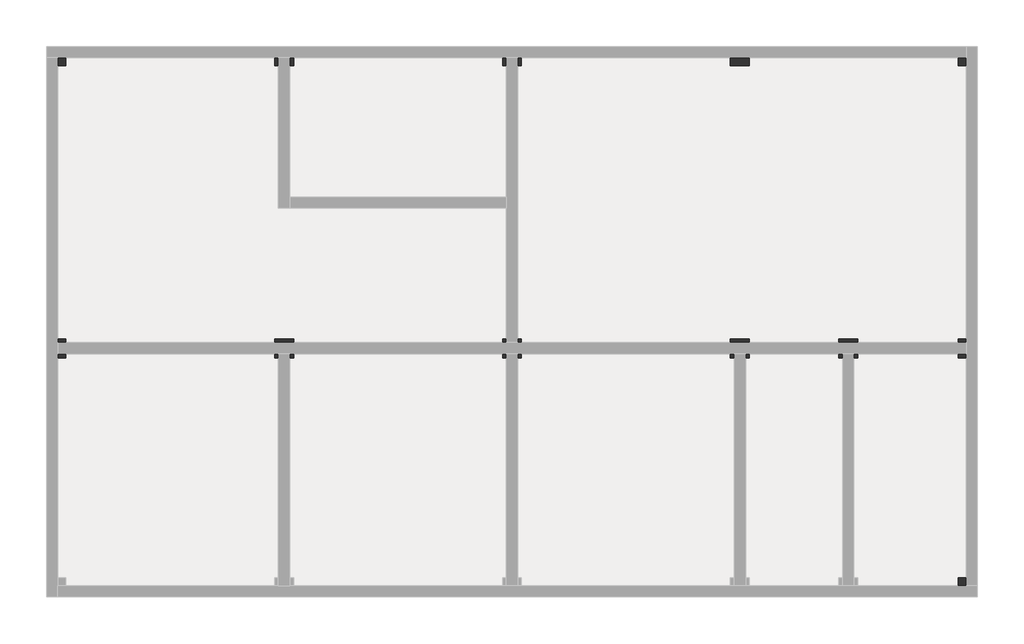
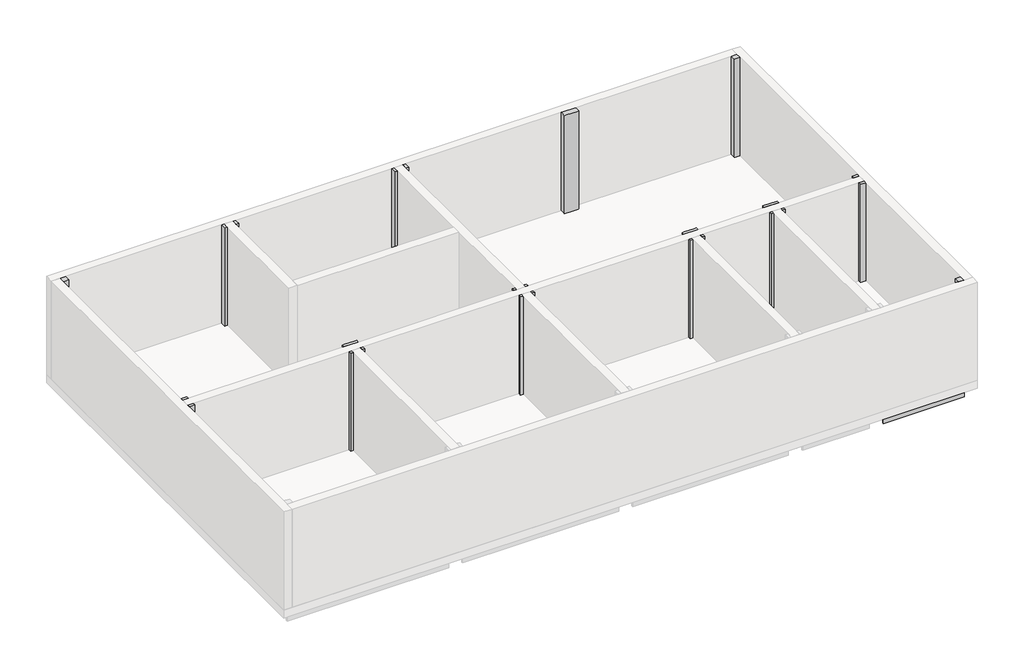
# One storey, part 2 of 2: 17 beams, 12 columns.
"""IFC4 building model written with IfcOpenShell, lengths in millimetres."""

from ifc_helpers import new_model, si_unit, frame, origin, place, context, project, spatial, polyline, outline, extrude, faceted_brep, element, save

model = new_model("IFC4")

# Units and contexts
model_context = context("Model", 3, world=origin())
ifc_project = project(units=[si_unit("LENGTHUNIT", "METRE", prefix="MILLI")], contexts=[model_context])

# Site, building, storey
site = spatial("IfcSite", under=ifc_project)
building = spatial("IfcBuilding", under=site)
storey = spatial("IfcBuildingStorey", under=building, Name="2nd FL GL+6,200", Elevation=6000.0)

# Beams
placement = place(None, origin())
element("IfcBeam", 1, ObjectType="RC Beam_Rectangular : 350 x 700mm", at=placement, inside=storey, context=model_context, shape_type="SweptSolid", body=[
    extrude(outline(polyline([(-18645.7273237, 9185.9763125), (-18595.7273237, 9185.9763125), (-18595.7273237, 1985.9763125), (-18645.7273237, 1985.9763125), (-18645.7273237, 9185.9763125)])), frame((0.0, 0.0, 5300.0), z_axis=(0.0, 0.0, 1.0), x_axis=(1.0, 0.0, 0.0)), (0.0, 0.0, 1.0), 400.0),
])
element("IfcBeam", 2, ObjectType="RC Beam_Rectangular : 350 x 700mm", at=placement, inside=storey, context=model_context, shape_type="SweptSolid", body=[
    extrude(outline(polyline([(-12870.7273237, 9185.9763125), (-12520.7273237, 9185.9763125), (-12520.7273237, 1985.9763125), (-12870.7273237, 1985.9763125), (-12870.7273237, 9185.9763125)])), frame((0.0, 0.0, 5300.0), z_axis=(0.0, 0.0, 1.0), x_axis=(1.0, 0.0, 0.0)), (0.0, 0.0, 1.0), 400.0),
])
element("IfcBeam", 3, ObjectType="RC Beam_Rectangular : 350 x 700mm", at=placement, inside=storey, context=model_context, shape_type="SweptSolid", body=[
    extrude(outline(polyline([(-6870.7273237, 9185.9763125), (-6520.7273237, 9185.9763125), (-6520.7273237, 1985.9763125), (-6870.7273237, 1985.9763125), (-6870.7273237, 9185.9763125)])), frame((0.0, 0.0, 5300.0), z_axis=(0.0, 0.0, 1.0), x_axis=(1.0, 0.0, 0.0)), (0.0, 0.0, 1.0), 400.0),
])
element("IfcBeam", 4, ObjectType="RC Beam_Rectangular : 350 x 700mm", at=placement, inside=storey, context=model_context, shape_type="SweptSolid", body=[
    extrude(outline(polyline([(-870.7273237, 9185.9763125), (-520.7273237, 9185.9763125), (-520.7273237, 1985.9763125), (-870.7273237, 1985.9763125), (-870.7273237, 9185.9763125)])), frame((0.0, 0.0, 5300.0), z_axis=(0.0, 0.0, 1.0), x_axis=(1.0, 0.0, 0.0)), (0.0, 0.0, 1.0), 400.0),
])
element("IfcBeam", 5, ObjectType="RC Beam_Rectangular : 350 x 700mm", at=placement, inside=storey, context=model_context, shape_type="SweptSolid", body=[
    extrude(outline(polyline([(5204.2726763, 1485.9763125), (5254.2726763, 1485.9763125), (5254.2726763, -4314.0236875), (5204.2726763, -4314.0236875), (5204.2726763, 1485.9763125)])), frame((0.0, 0.0, 5300.0), z_axis=(0.0, 0.0, 1.0), x_axis=(1.0, 0.0, 0.0)), (0.0, 0.0, 1.0), 400.0),
])
element("IfcBeam", 6, ObjectType="RC Beam_Rectangular : 350 x 700mm", at=placement, inside=storey, context=model_context, shape_type="SweptSolid", body=[
    extrude(outline(polyline([(5204.2726763, 9185.9763125), (5254.2726763, 9185.9763125), (5254.2726763, 1885.9763125), (5204.2726763, 1885.9763125), (5204.2726763, 9185.9763125)])), frame((0.0, 0.0, 5300.0), z_axis=(0.0, 0.0, 1.0), x_axis=(1.0, 0.0, 0.0)), (0.0, 0.0, 1.0), 400.0),
])
element("IfcBeam", 7, ObjectType="RC Beam_Rectangular : 350 x 700mm", at=placement, inside=storey, context=model_context, shape_type="SweptSolid", body=[
    extrude(outline(polyline([(-12945.7273237, 9385.9763125), (-12945.7273237, 9335.9763125), (-18645.7273237, 9335.9763125), (-18645.7273237, 9385.9763125), (-12945.7273237, 9385.9763125)])), frame((0.0, 0.0, 5300.0), z_axis=(0.0, 0.0, 1.0), x_axis=(1.0, 0.0, 0.0)), (0.0, 0.0, 1.0), 400.0),
])
element("IfcBeam", 8, ObjectType="RC Beam_Rectangular : 350 x 700mm", at=placement, inside=storey, context=model_context, shape_type="SweptSolid", body=[
    extrude(outline(polyline([(-12445.7273237, 9335.9763125), (-12445.7273237, 9385.9763125), (-6945.7273237, 9385.9763125), (-6945.7273237, 9335.9763125), (-12445.7273237, 9335.9763125)])), frame((0.0, 0.0, 5300.0), z_axis=(0.0, 0.0, 1.0), x_axis=(1.0, 0.0, 0.0)), (0.0, 0.0, 1.0), 400.0),
])
element("IfcBeam", 9, ObjectType="RC Beam_Rectangular : 350 x 700mm", at=placement, inside=storey, context=model_context, shape_type="SweptSolid", body=[
    extrude(outline(polyline([(-6445.7273237, 9335.9763125), (-6445.7273237, 9385.9763125), (-945.7273237, 9385.9763125), (-945.7273237, 9335.9763125), (-6445.7273237, 9335.9763125)])), frame((0.0, 0.0, 5300.0), z_axis=(0.0, 0.0, 1.0), x_axis=(1.0, 0.0, 0.0)), (0.0, 0.0, 1.0), 400.0),
])
element("IfcBeam", 10, ObjectType="RC Beam_Rectangular : 350 x 700mm", at=placement, inside=storey, context=model_context, shape_type="SweptSolid", body=[
    extrude(outline(polyline([(-433.0273237, 9385.9763125), (5254.2726763, 9385.9763125), (5254.2726763, 9335.9763125), (-433.0273237, 9335.9763125), (-433.0273237, 9385.9763125)])), frame((0.0, 0.0, 5300.0), z_axis=(0.0, 0.0, 1.0), x_axis=(1.0, 0.0, 0.0)), (0.0, 0.0, 1.0), 400.0),
])
element("IfcBeam", 11, ObjectType="RC Beam_Rectangular : 350 x 700mm", at=placement, inside=storey, context=model_context, shape_type="SweptSolid", body=[
    extrude(outline(polyline([(-18445.7273237, 1560.9763125), (-18445.7273237, 1585.9763125), (-12945.7273237, 1585.9763125), (-12945.7273237, 1560.9763125), (-18445.7273237, 1560.9763125)])), frame((0.0, 0.0, 5300.0), z_axis=(0.0, 0.0, 1.0), x_axis=(1.0, 0.0, 0.0)), (0.0, 0.0, 1.0), 400.0),
    extrude(outline(polyline([(-18445.7273237, 1885.9763125), (-18445.7273237, 1910.9763125), (-12945.7273237, 1910.9763125), (-12945.7273237, 1885.9763125), (-18445.7273237, 1885.9763125)])), frame((0.0, 0.0, 5300.0), z_axis=(0.0, 0.0, 1.0), x_axis=(1.0, 0.0, 0.0)), (0.0, 0.0, 1.0), 400.0),
])
element("IfcBeam", 12, ObjectType="RC Beam_Rectangular : 350 x 700mm", at=placement, inside=storey, context=model_context, shape_type="SweptSolid", body=[
    extrude(outline(polyline([(-12445.7273237, 1560.9763125), (-12445.7273237, 1585.9763125), (-6945.7273237, 1585.9763125), (-6945.7273237, 1560.9763125), (-12445.7273237, 1560.9763125)])), frame((0.0, 0.0, 5300.0), z_axis=(0.0, 0.0, 1.0), x_axis=(1.0, 0.0, 0.0)), (0.0, 0.0, 1.0), 400.0),
    extrude(outline(polyline([(-12445.7273237, 1885.9763125), (-12445.7273237, 1910.9763125), (-6945.7273237, 1910.9763125), (-6945.7273237, 1885.9763125), (-12445.7273237, 1885.9763125)])), frame((0.0, 0.0, 5300.0), z_axis=(0.0, 0.0, 1.0), x_axis=(1.0, 0.0, 0.0)), (0.0, 0.0, 1.0), 400.0),
])
element("IfcBeam", 13, ObjectType="RC Beam_Rectangular : 350 x 700mm", at=placement, inside=storey, context=model_context, shape_type="SweptSolid", body=[
    extrude(outline(polyline([(-6445.7273237, 1560.9763125), (-6445.7273237, 1585.9763125), (-945.7273237, 1585.9763125), (-945.7273237, 1560.9763125), (-6445.7273237, 1560.9763125)])), frame((0.0, 0.0, 5300.0), z_axis=(0.0, 0.0, 1.0), x_axis=(1.0, 0.0, 0.0)), (0.0, 0.0, 1.0), 400.0),
    extrude(outline(polyline([(-6445.7273237, 1885.9763125), (-6445.7273237, 1910.9763125), (-945.7273237, 1910.9763125), (-945.7273237, 1885.9763125), (-6445.7273237, 1885.9763125)])), frame((0.0, 0.0, 5300.0), z_axis=(0.0, 0.0, 1.0), x_axis=(1.0, 0.0, 0.0)), (0.0, 0.0, 1.0), 400.0),
])
element("IfcBeam", 14, ObjectType="RC Beam_Rectangular : 350 x 700mm", at=placement, inside=storey, context=model_context, shape_type="SweptSolid", body=[
    extrude(outline(polyline([(-445.7273237, 1560.9763125), (-445.7273237, 1585.9763125), (1904.2726763, 1585.9763125), (1904.2726763, 1560.9763125), (-445.7273237, 1560.9763125)])), frame((0.0, 0.0, 5300.0), z_axis=(0.0, 0.0, 1.0), x_axis=(1.0, 0.0, 0.0)), (0.0, 0.0, 1.0), 400.0),
    extrude(outline(polyline([(-445.7273237, 1885.9763125), (-445.7273237, 1910.9763125), (1904.2726763, 1910.9763125), (1904.2726763, 1885.9763125), (-445.7273237, 1885.9763125)])), frame((0.0, 0.0, 5300.0), z_axis=(0.0, 0.0, 1.0), x_axis=(1.0, 0.0, 0.0)), (0.0, 0.0, 1.0), 400.0),
])
element("IfcBeam", 15, ObjectType="RC Beam_Rectangular : 350 x 700mm", at=placement, inside=storey, context=model_context, shape_type="SweptSolid", body=[
    extrude(outline(polyline([(5054.2726763, 1585.9763125), (5054.2726763, 1560.9763125), (2404.2726763, 1560.9763125), (2404.2726763, 1585.9763125), (5054.2726763, 1585.9763125)])), frame((0.0, 0.0, 5300.0), z_axis=(0.0, 0.0, 1.0), x_axis=(1.0, 0.0, 0.0)), (0.0, 0.0, 1.0), 400.0),
    extrude(outline(polyline([(5054.2726763, 1910.9763125), (5054.2726763, 1885.9763125), (2404.2726763, 1885.9763125), (2404.2726763, 1910.9763125), (5054.2726763, 1910.9763125)])), frame((0.0, 0.0, 5300.0), z_axis=(0.0, 0.0, 1.0), x_axis=(1.0, 0.0, 0.0)), (0.0, 0.0, 1.0), 400.0),
])
element("IfcBeam", 16, ObjectType="RC Beam_Rectangular : 350 x 700mm", at=placement, inside=storey, context=model_context, shape_type="SweptSolid", body=[
    extrude(outline(polyline([(2404.2726763, -4514.0236875), (2404.2726763, -4464.0236875), (5254.2726763, -4464.0236875), (5254.2726763, -4514.0236875), (2404.2726763, -4514.0236875)])), frame((0.0, 0.0, 5300.0), z_axis=(0.0, 0.0, 1.0), x_axis=(1.0, 0.0, 0.0)), (0.0, 0.0, 1.0), 400.0),
])
element("IfcBeam", 17, ObjectType="RC Beam_Rectangular : 350 x 700mm", at=placement, inside=storey, context=model_context, shape_type="SweptSolid", body=[
    extrude(outline(polyline([(2304.2726763, 1485.9763125), (2329.2726763, 1485.9763125), (2329.2726763, -4314.0236875), (2304.2726763, -4314.0236875), (2304.2726763, 1485.9763125)])), frame((0.0, 0.0, 5300.0), z_axis=(0.0, 0.0, 1.0), x_axis=(1.0, 0.0, 0.0)), (0.0, 0.0, 1.0), 400.0),
    extrude(outline(polyline([(1979.2726763, 1485.9763125), (2004.2726763, 1485.9763125), (2004.2726763, -4314.0236875), (1979.2726763, -4314.0236875), (1979.2726763, 1485.9763125)])), frame((0.0, 0.0, 5300.0), z_axis=(0.0, 0.0, 1.0), x_axis=(1.0, 0.0, 0.0)), (0.0, 0.0, 1.0), 400.0),
])

# Columns
element("IfcColumn", 18, ObjectType="RC_Column_Rectangular : 500 x 500mm", at=placement, inside=storey, context=model_context, shape_type="Brep", body=[
    faceted_brep([(-18445.7273237, 9385.9763125, 6000.0), (-18445.7273237, 9185.9763125, 6000.0), (-18645.7273237, 9185.9763125, 6000.0), (-18645.7273237, 9385.9763125, 6000.0), (-18445.7273237, 9185.9763125, 9667.0), (-18595.7273237, 9185.9763125, 9667.0), (-18645.7273237, 9185.9763125, 9667.0), (-18645.7273237, 9185.9763125, 9300.0), (-18445.7273237, 9385.9763125, 9300.0), (-18445.7273237, 9385.9763125, 9667.0), (-18445.7273237, 9335.9763125, 9667.0), (-18645.7273237, 9385.9763125, 9667.0)], [[[0, 1, 2, 3]], [[1, 4, 5, 6, 7, 2]], [[4, 1, 0, 8, 9, 10]], [[4, 10, 9, 11, 6, 5]], [[9, 8, 0, 3, 11]], [[3, 2, 7, 6, 11]]]),
])
element("IfcColumn", 19, ObjectType="RC_Column_Rectangular : 500 x 500mm", at=placement, inside=storey, context=model_context, shape_type="Brep", body=[
    faceted_brep([(-18645.7273237, 1985.9763125, 6000.0), (-18445.7273237, 1985.9763125, 6000.0), (-18445.7273237, 1885.9763125, 6000.0), (-18645.7273237, 1885.9763125, 6000.0), (-18445.7273237, 1985.9763125, 9667.0), (-18645.7273237, 1985.9763125, 9300.0), (-18645.7273237, 1985.9763125, 9667.0), (-18595.7273237, 1985.9763125, 9667.0), (-18445.7273237, 1910.9763125, 9667.0), (-18445.7273237, 1885.9763125, 9667.0), (-18445.7273237, 1885.9763125, 9300.0), (-18645.7273237, 1885.9763125, 9667.0)], [[[0, 1, 2, 3]], [[4, 1, 0, 5, 6, 7]], [[1, 4, 8, 9, 10, 2]], [[4, 7, 6, 11, 9, 8]], [[3, 2, 10, 9, 11]], [[6, 5, 0, 3, 11]]]),
    faceted_brep([(-18445.7273237, 1485.9763125, 6000.0), (-18445.7273237, 1485.9763125, 9667.0), (-18595.7273237, 1485.9763125, 9667.0), (-18645.7273237, 1485.9763125, 9667.0), (-18645.7273237, 1485.9763125, 9300.0), (-18645.7273237, 1485.9763125, 6000.0), (-18645.7273237, 1585.9763125, 9667.0), (-18645.7273237, 1585.9763125, 6000.0), (-18445.7273237, 1585.9763125, 6000.0), (-18445.7273237, 1585.9763125, 9667.0), (-18445.7273237, 1585.9763125, 9300.0), (-18445.7273237, 1560.9763125, 9667.0)], [[[0, 1, 2, 3, 4, 5]], [[5, 4, 3, 6, 7]], [[8, 7, 6, 9, 10]], [[0, 5, 7, 8]], [[1, 0, 8, 10, 9, 11]], [[3, 2, 1, 11, 9, 6]]]),
])
element("IfcColumn", 20, ObjectType="RC_Column_Rectangular : 500 x 500mm", at=placement, inside=storey, context=model_context, shape_type="Brep", body=[
    faceted_brep([(-12945.7273237, 9185.9763125, 6000.0), (-12945.7273237, 9385.9763125, 6000.0), (-12845.7273237, 9385.9763125, 6000.0), (-12845.7273237, 9185.9763125, 6000.0), (-12945.7273237, 9185.9763125, 9667.0), (-12945.7273237, 9335.9763125, 9667.0), (-12945.7273237, 9385.9763125, 9667.0), (-12945.7273237, 9385.9763125, 9300.0), (-12845.7273237, 9185.9763125, 9300.0), (-12845.7273237, 9185.9763125, 9667.0), (-12870.7273237, 9185.9763125, 9667.0), (-12845.7273237, 9385.9763125, 9667.0)], [[[0, 1, 2, 3]], [[0, 4, 5, 6, 7, 1]], [[4, 0, 3, 8, 9, 10]], [[6, 5, 4, 10, 9, 11]], [[1, 7, 6, 11, 2]], [[3, 2, 11, 9, 8]]]),
    faceted_brep([(-12445.7273237, 9185.9763125, 9667.0), (-12445.7273237, 9185.9763125, 6000.0), (-12445.7273237, 9385.9763125, 6000.0), (-12445.7273237, 9385.9763125, 9300.0), (-12445.7273237, 9385.9763125, 9667.0), (-12445.7273237, 9335.9763125, 9667.0), (-12545.7273237, 9385.9763125, 6000.0), (-12545.7273237, 9185.9763125, 6000.0), (-12545.7273237, 9185.9763125, 9300.0), (-12545.7273237, 9185.9763125, 9667.0), (-12545.7273237, 9385.9763125, 9667.0), (-12520.7273237, 9185.9763125, 9667.0)], [[[0, 1, 2, 3, 4, 5]], [[6, 7, 8, 9, 10]], [[2, 1, 7, 6]], [[1, 0, 11, 9, 8, 7]], [[0, 5, 4, 10, 9, 11]], [[4, 3, 2, 6, 10]]]),
])
element("IfcColumn", 21, ObjectType="RC_Column_Rectangular : 500 x 500mm", at=placement, inside=storey, context=model_context, shape_type="Brep", body=[
    faceted_brep([(-12945.7273237, 1985.9763125, 6000.0), (-12445.7273237, 1985.9763125, 6000.0), (-12445.7273237, 1885.9763125, 6000.0), (-12945.7273237, 1885.9763125, 6000.0), (-12945.7273237, 1985.9763125, 9667.0), (-12870.7273237, 1985.9763125, 9667.0), (-12520.7273237, 1985.9763125, 9667.0), (-12445.7273237, 1985.9763125, 9667.0), (-12945.7273237, 1885.9763125, 9300.0), (-12945.7273237, 1885.9763125, 9667.0), (-12945.7273237, 1910.9763125, 9667.0), (-12445.7273237, 1910.9763125, 9667.0), (-12445.7273237, 1885.9763125, 9667.0), (-12445.7273237, 1885.9763125, 9300.0)], [[[0, 1, 2, 3]], [[1, 0, 4, 5, 6, 7]], [[4, 0, 3, 8, 9, 10]], [[1, 7, 11, 12, 13, 2]], [[7, 6, 5, 4, 10, 9, 12, 11]], [[3, 2, 13, 12, 9, 8]]]),
    faceted_brep([(-12945.7273237, 1485.9763125, 9667.0), (-12945.7273237, 1485.9763125, 6000.0), (-12845.7273237, 1485.9763125, 6000.0), (-12845.7273237, 1485.9763125, 9300.0), (-12845.7273237, 1485.9763125, 9667.0), (-12870.7273237, 1485.9763125, 9667.0), (-12945.7273237, 1585.9763125, 6000.0), (-12945.7273237, 1585.9763125, 9300.0), (-12945.7273237, 1585.9763125, 9667.0), (-12845.7273237, 1585.9763125, 9667.0), (-12845.7273237, 1585.9763125, 6000.0), (-12945.7273237, 1560.9763125, 9667.0)], [[[0, 1, 2, 3, 4, 5]], [[6, 7, 8, 9, 10]], [[1, 6, 10, 2]], [[1, 0, 11, 8, 7, 6]], [[8, 11, 0, 5, 4, 9]], [[4, 3, 2, 10, 9]]]),
    faceted_brep([(-12445.7273237, 1485.9763125, 9667.0), (-12445.7273237, 1485.9763125, 6000.0), (-12445.7273237, 1585.9763125, 6000.0), (-12445.7273237, 1585.9763125, 9300.0), (-12445.7273237, 1585.9763125, 9667.0), (-12445.7273237, 1560.9763125, 9667.0), (-12545.7273237, 1485.9763125, 6000.0), (-12545.7273237, 1485.9763125, 9300.0), (-12545.7273237, 1485.9763125, 9667.0), (-12545.7273237, 1585.9763125, 9667.0), (-12545.7273237, 1585.9763125, 6000.0), (-12520.7273237, 1485.9763125, 9667.0)], [[[0, 1, 2, 3, 4, 5]], [[6, 7, 8, 9, 10]], [[1, 0, 11, 8, 7, 6]], [[4, 3, 2, 10, 9]], [[2, 1, 6, 10]], [[0, 5, 4, 9, 8, 11]]]),
])
element("IfcColumn", 22, ObjectType="RC_Column_Rectangular : 500 x 500mm", at=placement, inside=storey, context=model_context, shape_type="Brep", body=[
    faceted_brep([(-6945.7273237, 9185.9763125, 6000.0), (-6945.7273237, 9385.9763125, 6000.0), (-6845.7273237, 9385.9763125, 6000.0), (-6845.7273237, 9185.9763125, 6000.0), (-6945.7273237, 9185.9763125, 9667.0), (-6945.7273237, 9335.9763125, 9667.0), (-6945.7273237, 9385.9763125, 9667.0), (-6945.7273237, 9385.9763125, 9300.0), (-6845.7273237, 9185.9763125, 9300.0), (-6845.7273237, 9185.9763125, 9667.0), (-6870.7273237, 9185.9763125, 9667.0), (-6845.7273237, 9385.9763125, 9667.0)], [[[0, 1, 2, 3]], [[0, 4, 5, 6, 7, 1]], [[4, 0, 3, 8, 9, 10]], [[6, 5, 4, 10, 9, 11]], [[1, 7, 6, 11, 2]], [[3, 2, 11, 9, 8]]]),
    faceted_brep([(-6445.7273237, 9185.9763125, 9667.0), (-6445.7273237, 9185.9763125, 6000.0), (-6445.7273237, 9385.9763125, 6000.0), (-6445.7273237, 9385.9763125, 9300.0), (-6445.7273237, 9385.9763125, 9667.0), (-6445.7273237, 9335.9763125, 9667.0), (-6545.7273237, 9385.9763125, 6000.0), (-6545.7273237, 9185.9763125, 6000.0), (-6545.7273237, 9185.9763125, 9300.0), (-6545.7273237, 9185.9763125, 9667.0), (-6545.7273237, 9385.9763125, 9667.0), (-6520.7273237, 9185.9763125, 9667.0)], [[[0, 1, 2, 3, 4, 5]], [[6, 7, 8, 9, 10]], [[2, 1, 7, 6]], [[1, 0, 11, 9, 8, 7]], [[0, 5, 4, 10, 9, 11]], [[4, 3, 2, 6, 10]]]),
])
element("IfcColumn", 23, ObjectType="RC_Column_Rectangular : 500 x 500mm", at=placement, inside=storey, context=model_context, shape_type="Brep", body=[
    faceted_brep([(-6945.7273237, 1985.9763125, 6000.0), (-6845.7273237, 1985.9763125, 6000.0), (-6845.7273237, 1885.9763125, 6000.0), (-6945.7273237, 1885.9763125, 6000.0), (-6945.7273237, 1985.9763125, 9667.0), (-6945.7273237, 1885.9763125, 9300.0), (-6945.7273237, 1885.9763125, 9667.0), (-6945.7273237, 1910.9763125, 9667.0), (-6845.7273237, 1985.9763125, 9667.0), (-6870.7273237, 1985.9763125, 9667.0), (-6845.7273237, 1885.9763125, 9667.0), (-6845.7273237, 1985.9763125, 9300.0)], [[[0, 1, 2, 3]], [[4, 0, 3, 5, 6, 7]], [[8, 9, 4, 7, 6, 10]], [[2, 1, 11, 8, 10]], [[0, 4, 9, 8, 11, 1]], [[3, 2, 10, 6, 5]]]),
    faceted_brep([(-6445.7273237, 1985.9763125, 9667.0), (-6445.7273237, 1985.9763125, 6000.0), (-6545.7273237, 1985.9763125, 6000.0), (-6545.7273237, 1985.9763125, 9300.0), (-6545.7273237, 1985.9763125, 9667.0), (-6520.7273237, 1985.9763125, 9667.0), (-6445.7273237, 1910.9763125, 9667.0), (-6445.7273237, 1885.9763125, 9667.0), (-6445.7273237, 1885.9763125, 9300.0), (-6445.7273237, 1885.9763125, 6000.0), (-6545.7273237, 1885.9763125, 6000.0), (-6545.7273237, 1885.9763125, 9667.0)], [[[0, 1, 2, 3, 4, 5]], [[1, 0, 6, 7, 8, 9]], [[2, 10, 11, 4, 3]], [[10, 9, 8, 7, 11]], [[2, 1, 9, 10]], [[0, 5, 4, 11, 7, 6]]]),
    faceted_brep([(-6945.7273237, 1485.9763125, 9667.0), (-6945.7273237, 1485.9763125, 6000.0), (-6845.7273237, 1485.9763125, 6000.0), (-6845.7273237, 1485.9763125, 9300.0), (-6845.7273237, 1485.9763125, 9667.0), (-6870.7273237, 1485.9763125, 9667.0), (-6945.7273237, 1585.9763125, 6000.0), (-6945.7273237, 1585.9763125, 9300.0), (-6945.7273237, 1585.9763125, 9667.0), (-6845.7273237, 1585.9763125, 9667.0), (-6845.7273237, 1585.9763125, 6000.0), (-6945.7273237, 1560.9763125, 9667.0)], [[[0, 1, 2, 3, 4, 5]], [[6, 7, 8, 9, 10]], [[1, 6, 10, 2]], [[1, 0, 11, 8, 7, 6]], [[8, 11, 0, 5, 4, 9]], [[4, 3, 2, 10, 9]]]),
    faceted_brep([(-6445.7273237, 1485.9763125, 9667.0), (-6445.7273237, 1485.9763125, 6000.0), (-6445.7273237, 1585.9763125, 6000.0), (-6445.7273237, 1585.9763125, 9300.0), (-6445.7273237, 1585.9763125, 9667.0), (-6445.7273237, 1560.9763125, 9667.0), (-6545.7273237, 1485.9763125, 6000.0), (-6545.7273237, 1485.9763125, 9300.0), (-6545.7273237, 1485.9763125, 9667.0), (-6545.7273237, 1585.9763125, 9667.0), (-6545.7273237, 1585.9763125, 6000.0), (-6520.7273237, 1485.9763125, 9667.0)], [[[0, 1, 2, 3, 4, 5]], [[6, 7, 8, 9, 10]], [[1, 0, 11, 8, 7, 6]], [[4, 3, 2, 10, 9]], [[2, 1, 6, 10]], [[0, 5, 4, 9, 8, 11]]]),
])
element("IfcColumn", 24, ObjectType="RC_Column_Rectangular : 500 x 500mm", at=placement, inside=storey, context=model_context, shape_type="Brep", body=[
    faceted_brep([(-445.7273237, 9185.9763125, 6000.0), (-945.7273237, 9185.9763125, 6000.0), (-945.7273237, 9385.9763125, 6000.0), (-445.7273237, 9385.9763125, 6000.0), (-945.7273237, 9185.9763125, 9667.0), (-945.7273237, 9335.9763125, 9667.0), (-945.7273237, 9385.9763125, 9667.0), (-945.7273237, 9385.9763125, 9300.0), (-445.7273237, 9185.9763125, 9667.0), (-520.7273237, 9185.9763125, 9667.0), (-870.7273237, 9185.9763125, 9667.0), (-445.7273237, 9385.9763125, 9300.0), (-445.7273237, 9385.9763125, 9667.0), (-445.7273237, 9335.9763125, 9667.0)], [[[0, 1, 2, 3]], [[1, 4, 5, 6, 7, 2]], [[1, 0, 8, 9, 10, 4]], [[8, 0, 3, 11, 12, 13]], [[4, 10, 9, 8, 13, 12, 6, 5]], [[3, 2, 7, 6, 12, 11]]]),
])
element("IfcColumn", 25, ObjectType="RC_Column_Rectangular : 500 x 500mm", at=placement, inside=storey, context=model_context, shape_type="Brep", body=[
    faceted_brep([(-945.7273237, 1985.9763125, 6000.0), (-445.7273237, 1985.9763125, 6000.0), (-445.7273237, 1885.9763125, 6000.0), (-945.7273237, 1885.9763125, 6000.0), (-945.7273237, 1985.9763125, 9667.0), (-870.7273237, 1985.9763125, 9667.0), (-520.7273237, 1985.9763125, 9667.0), (-445.7273237, 1985.9763125, 9667.0), (-945.7273237, 1885.9763125, 9300.0), (-945.7273237, 1885.9763125, 9667.0), (-945.7273237, 1910.9763125, 9667.0), (-445.7273237, 1910.9763125, 9667.0), (-445.7273237, 1885.9763125, 9667.0), (-445.7273237, 1885.9763125, 9300.0)], [[[0, 1, 2, 3]], [[1, 0, 4, 5, 6, 7]], [[4, 0, 3, 8, 9, 10]], [[1, 7, 11, 12, 13, 2]], [[7, 6, 5, 4, 10, 9, 12, 11]], [[3, 2, 13, 12, 9, 8]]]),
    faceted_brep([(-945.7273237, 1485.9763125, 9667.0), (-945.7273237, 1485.9763125, 6000.0), (-845.7273237, 1485.9763125, 6000.0), (-845.7273237, 1485.9763125, 9300.0), (-845.7273237, 1485.9763125, 9667.0), (-870.7273237, 1485.9763125, 9667.0), (-945.7273237, 1585.9763125, 6000.0), (-945.7273237, 1585.9763125, 9300.0), (-945.7273237, 1585.9763125, 9667.0), (-845.7273237, 1585.9763125, 9667.0), (-845.7273237, 1585.9763125, 6000.0), (-945.7273237, 1560.9763125, 9667.0)], [[[0, 1, 2, 3, 4, 5]], [[6, 7, 8, 9, 10]], [[1, 6, 10, 2]], [[1, 0, 11, 8, 7, 6]], [[8, 11, 0, 5, 4, 9]], [[4, 3, 2, 10, 9]]]),
    faceted_brep([(-445.7273237, 1485.9763125, 9667.0), (-445.7273237, 1485.9763125, 6000.0), (-445.7273237, 1585.9763125, 6000.0), (-445.7273237, 1585.9763125, 9300.0), (-445.7273237, 1585.9763125, 9667.0), (-445.7273237, 1560.9763125, 9667.0), (-545.7273237, 1485.9763125, 6000.0), (-545.7273237, 1485.9763125, 9300.0), (-545.7273237, 1485.9763125, 9667.0), (-545.7273237, 1585.9763125, 9667.0), (-545.7273237, 1585.9763125, 6000.0), (-520.7273237, 1485.9763125, 9667.0)], [[[0, 1, 2, 3, 4, 5]], [[6, 7, 8, 9, 10]], [[1, 0, 11, 8, 7, 6]], [[4, 3, 2, 10, 9]], [[2, 1, 6, 10]], [[0, 5, 4, 9, 8, 11]]]),
])
element("IfcColumn", 26, ObjectType="RC_Column_Rectangular : 500 x 500mm", at=placement, inside=storey, context=model_context, shape_type="Brep", body=[
    faceted_brep([(5054.2726763, 9185.9763125, 6000.0), (5054.2726763, 9385.9763125, 6000.0), (5254.2726763, 9385.9763125, 6000.0), (5254.2726763, 9185.9763125, 6000.0), (5054.2726763, 9185.9763125, 9667.0), (5054.2726763, 9385.9763125, 9667.0), (5254.2726763, 9185.9763125, 9300.0), (5254.2726763, 9185.9763125, 9667.0), (5204.2726763, 9185.9763125, 9667.0), (5254.2726763, 9385.9763125, 9667.0)], [[[0, 1, 2, 3]], [[0, 4, 5, 1]], [[4, 0, 3, 6, 7, 8]], [[5, 4, 8, 7, 9]], [[2, 1, 5, 9]], [[3, 2, 9, 7, 6]]]),
])
element("IfcColumn", 27, ObjectType="RC_Column_Rectangular : 500 x 500mm", at=placement, inside=storey, context=model_context, shape_type="Brep", body=[
    faceted_brep([(5054.2726763, 1985.9763125, 6000.0), (5254.2726763, 1985.9763125, 6000.0), (5254.2726763, 1885.9763125, 6000.0), (5054.2726763, 1885.9763125, 6000.0), (5054.2726763, 1985.9763125, 9667.0), (5254.2726763, 1985.9763125, 9667.0), (5054.2726763, 1885.9763125, 9300.0), (5054.2726763, 1885.9763125, 9667.0), (5054.2726763, 1910.9763125, 9667.0), (5254.2726763, 1885.9763125, 9667.0)], [[[0, 1, 2, 3]], [[0, 4, 5, 1]], [[4, 0, 3, 6, 7, 8]], [[5, 4, 8, 7, 9]], [[1, 5, 9, 2]], [[3, 2, 9, 7, 6]]]),
    faceted_brep([(5054.2726763, 1485.9763125, 9667.0), (5054.2726763, 1485.9763125, 6000.0), (5254.2726763, 1485.9763125, 6000.0), (5254.2726763, 1485.9763125, 9300.0), (5254.2726763, 1485.9763125, 9667.0), (5204.2726763, 1485.9763125, 9667.0), (5254.2726763, 1585.9763125, 6000.0), (5054.2726763, 1585.9763125, 6000.0), (5054.2726763, 1585.9763125, 9300.0), (5054.2726763, 1585.9763125, 9667.0), (5254.2726763, 1585.9763125, 9667.0), (5054.2726763, 1560.9763125, 9667.0)], [[[0, 1, 2, 3, 4, 5]], [[6, 7, 8, 9, 10]], [[2, 1, 7, 6]], [[1, 0, 11, 9, 8, 7]], [[0, 5, 4, 10, 9, 11]], [[4, 3, 2, 6, 10]]]),
])
element("IfcColumn", 28, ObjectType="RC_Column_Rectangular : 500 x 500mm", at=placement, inside=storey, context=model_context, shape_type="Brep", body=[
    faceted_brep([(5054.2726763, -4514.0236875, 6000.0), (5054.2726763, -4314.0236875, 6000.0), (5254.2726763, -4314.0236875, 6000.0), (5254.2726763, -4514.0236875, 6000.0), (5054.2726763, -4314.0236875, 9667.0), (5204.2726763, -4314.0236875, 9667.0), (5254.2726763, -4314.0236875, 9667.0), (5254.2726763, -4314.0236875, 9300.0), (5054.2726763, -4514.0236875, 9300.0), (5054.2726763, -4514.0236875, 9667.0), (5054.2726763, -4464.0236875, 9667.0), (5254.2726763, -4514.0236875, 9667.0)], [[[0, 1, 2, 3]], [[1, 4, 5, 6, 7, 2]], [[4, 1, 0, 8, 9, 10]], [[4, 10, 9, 11, 6, 5]], [[9, 8, 0, 3, 11]], [[3, 2, 7, 6, 11]]]),
])
element("IfcColumn", 29, ObjectType="RC_Column_Rectangular : 500 x 500mm", at=placement, inside=storey, context=model_context, shape_type="Brep", body=[
    faceted_brep([(1904.2726763, 1985.9763125, 6000.0), (2404.2726763, 1985.9763125, 6000.0), (2404.2726763, 1885.9763125, 6000.0), (1904.2726763, 1885.9763125, 6000.0), (1904.2726763, 1985.9763125, 9667.0), (2404.2726763, 1985.9763125, 9667.0), (1904.2726763, 1885.9763125, 9300.0), (1904.2726763, 1885.9763125, 9667.0), (1904.2726763, 1910.9763125, 9667.0), (2404.2726763, 1910.9763125, 9667.0), (2404.2726763, 1885.9763125, 9667.0), (2404.2726763, 1885.9763125, 9300.0)], [[[0, 1, 2, 3]], [[1, 0, 4, 5]], [[4, 0, 3, 6, 7, 8]], [[1, 5, 9, 10, 11, 2]], [[5, 4, 8, 7, 10, 9]], [[3, 2, 11, 10, 7, 6]]]),
    faceted_brep([(1904.2726763, 1485.9763125, 9667.0), (1904.2726763, 1485.9763125, 6000.0), (2004.2726763, 1485.9763125, 6000.0), (2004.2726763, 1485.9763125, 9300.0), (2004.2726763, 1485.9763125, 9667.0), (1979.2726763, 1485.9763125, 9667.0), (1904.2726763, 1585.9763125, 6000.0), (1904.2726763, 1585.9763125, 9300.0), (1904.2726763, 1585.9763125, 9667.0), (2004.2726763, 1585.9763125, 9667.0), (2004.2726763, 1585.9763125, 6000.0), (1904.2726763, 1560.9763125, 9667.0)], [[[0, 1, 2, 3, 4, 5]], [[6, 7, 8, 9, 10]], [[1, 6, 10, 2]], [[1, 0, 11, 8, 7, 6]], [[8, 11, 0, 5, 4, 9]], [[4, 3, 2, 10, 9]]]),
    faceted_brep([(2404.2726763, 1485.9763125, 9667.0), (2404.2726763, 1485.9763125, 6000.0), (2404.2726763, 1585.9763125, 6000.0), (2404.2726763, 1585.9763125, 9300.0), (2404.2726763, 1585.9763125, 9667.0), (2404.2726763, 1560.9763125, 9667.0), (2304.2726763, 1485.9763125, 6000.0), (2304.2726763, 1485.9763125, 9300.0), (2304.2726763, 1485.9763125, 9667.0), (2304.2726763, 1585.9763125, 9667.0), (2304.2726763, 1585.9763125, 6000.0), (2329.2726763, 1485.9763125, 9667.0)], [[[0, 1, 2, 3, 4, 5]], [[6, 7, 8, 9, 10]], [[1, 0, 11, 8, 7, 6]], [[4, 3, 2, 10, 9]], [[2, 1, 6, 10]], [[0, 5, 4, 9, 8, 11]]]),
])

save(model, "model.ifc")

# Revit data of these elements
# Type "RC Beam_Rectangular : 350 x 700mm"
#   Length [instance default] = 1524 mm
#   b = 350 mm
#   h = 700 mm
#   Structural Material [instance default] = 콘크리트, 현장타설 회색
#   Assembly Code = ""
# Type "RC_Column_Rectangular : 500 x 500mm"
#   b = 500 mm
#   h = 500 mm
#   Structural Material [instance default] = 콘크리트, 현장타설 회색
# Elements 1, 2, 3, 4, 5, 6, 7, 8, 9, 10, 11, 12, 13, 14, 15, 16, 17 (IfcBeam, "RC Beam_Rectangular : 350 x 700mm")
#   Structural Material = 콘크리트, 현장타설 회색
#   Phase Created = 신축
#   Materials on its faces: "콘크리트, 현장타설 회색"
# Elements 18, 19, 20, 21, 22, 23, 24, 25, 26, 27, 28, 29 (IfcColumn, "RC_Column_Rectangular : 500 x 500mm")
#   Structural Material = 콘크리트, 현장타설 회색
#   Phase Created = 신축
#   Materials on its faces: "콘크리트, 현장타설 회색"
# Materials
#   "콘크리트, 현장타설 회색": class "콘크리트", colour RGB 192 192 192, transparency 0, Description = "현장타설 콘크리트", Cost = 0
